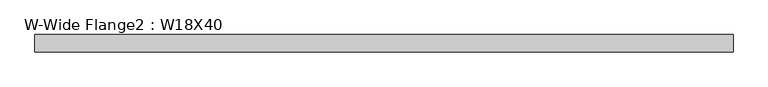
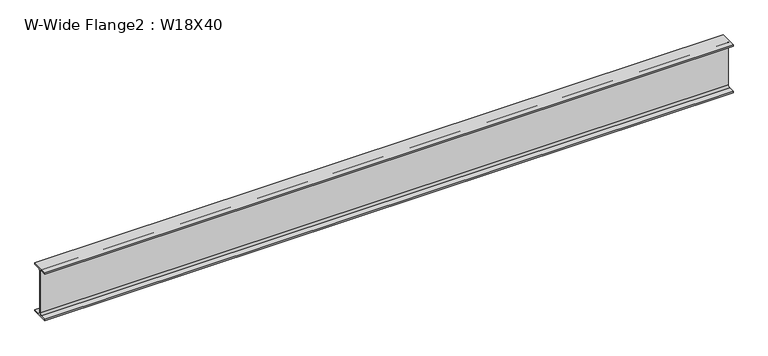
"""IFC4 building model written with IfcOpenShell, lengths in millimetres: beam geometry, W-Wide Flange2 : W18X40."""

import ifcopenshell
import ifcopenshell.guid

model = None  # the IFC model being written
_history = None  # IfcOwnerHistory: only IFC2X3 demands one
_inside = {}  # id of a spatial element -> (the spatial element, [elements in it])
_under = {}  # id of a project, library or spatial element -> (it, [spatial elements below it])
_declared = {}  # id of a project -> (the project, [libraries it declares])
_typed = {}  # id of a type object -> (the type object, [elements of that type])
_made_of = {}  # id of a material, layer set ... -> (it, [elements and type objects made of it])


def new_model(schema):
    """Start an empty IFC model of exactly this schema.

    Asked for "IFC4X3", IfcOpenShell would pick the latest addendum, in which some entities
    have other attributes; the version numbers below select the first issue.
    IFC2X3 requires an IfcOwnerHistory on every rooted entity: one is made here for all.
    """
    global model, _history
    if schema == "IFC4X3":
        model = ifcopenshell.file(schema_version=(4, 3, 0, 0))
    else:
        model = ifcopenshell.file(schema=schema)
    _inside.clear()
    _under.clear()
    _declared.clear()
    _typed.clear()
    _made_of.clear()
    _history = None
    if model.schema == "IFC2X3":
        org = make("IfcOrganization", Name="unknown")
        user = make(
            "IfcPersonAndOrganization",
            ThePerson=make("IfcPerson", FamilyName="unknown"),
            TheOrganization=org,
        )
        app = make(
            "IfcApplication",
            ApplicationDeveloper=org,
            Version="unknown",
            ApplicationFullName="unknown",
            ApplicationIdentifier="unknown",
        )
        _history = make(
            "IfcOwnerHistory",
            OwningUser=user,
            OwningApplication=app,
            ChangeAction="ADDED",
            CreationDate=0,
        )
    return model


def make(cls, **values):
    """One entity of the class cls with the attributes given. An attribute that is None is left unset."""
    return model.create_entity(
        cls, **{name: value for name, value in values.items() if value is not None}
    )


def rooted(cls, **values):
    """An entity with a GlobalId (a new one), such as an element, a storey or a relation."""
    return make(cls, GlobalId=ifcopenshell.guid.new(), OwnerHistory=_history, **values)


def si_unit(unit_type, name, prefix=None):
    """IfcSIUnit, for example si_unit("LENGTHUNIT", "METRE", prefix="MILLI")."""
    return make("IfcSIUnit", UnitType=unit_type, Prefix=prefix, Name=name)


def assignment(units):
    """IfcUnitAssignment: the units of a project."""
    return None if units is None else make("IfcUnitAssignment", Units=units)


def point(xyz):
    """IfcCartesianPoint."""
    return None if xyz is None else make("IfcCartesianPoint", Coordinates=xyz)


def direction(xyz):
    """IfcDirection."""
    return None if xyz is None else make("IfcDirection", DirectionRatios=xyz)


def frame(location, z_axis=None, x_axis=None):
    """IfcAxis2Placement3D, a coordinate frame: its origin and axes. An axis left out is left unset."""
    return make(
        "IfcAxis2Placement3D",
        Location=point(location),
        Axis=direction(z_axis),
        RefDirection=direction(x_axis),
    )


def frame_2d(location, x_axis=None):
    """IfcAxis2Placement2D, a coordinate frame in the plane: its origin and x axis."""
    return make(
        "IfcAxis2Placement2D", Location=point(location), RefDirection=direction(x_axis)
    )


def origin():
    """The frame at (0, 0, 0) with its axes left unset."""
    return frame((0.0, 0.0, 0.0))


def place(relative_to, where):
    """IfcLocalPlacement: puts the frame where relative to a parent placement (None: the world)."""
    return make(
        "IfcLocalPlacement", PlacementRelTo=relative_to, RelativePlacement=where
    )


def context(
    kind, dimensions, precision=None, world=None, true_north=None, identifier=None
):
    """IfcGeometricRepresentationContext, for example the 3D "Model" context."""
    return make(
        "IfcGeometricRepresentationContext",
        ContextIdentifier=identifier,
        ContextType=kind,
        CoordinateSpaceDimension=dimensions,
        Precision=precision,
        WorldCoordinateSystem=world,
        TrueNorth=true_north,
    )


def project(units=None, contexts=None):
    """IfcProject with its units and contexts."""
    return rooted(
        "IfcProject",
        Name="project",
        RepresentationContexts=contexts,
        UnitsInContext=assignment(units),
    )


def spatial(cls, under=None, at=None, **own):
    """A site, building, storey or space (cls), placed at a placement, below another one or the project."""
    s = rooted(cls, ObjectPlacement=at, **own)
    if under is not None:
        _under.setdefault(under.id(), (under, []))[1].append(s)
    return s


def polyline(points):
    """IfcPolyline through the points."""
    return make("IfcPolyline", Points=[point(p) for p in points])


def circle_curve(where, radius):
    """IfcCircle in the frame where."""
    return make("IfcCircle", Position=where, Radius=radius)


def trimmed(basis, trim1, trim2, sense, master):
    """IfcTrimmedCurve: the piece of a basis curve between two trims."""
    return make(
        "IfcTrimmedCurve",
        BasisCurve=basis,
        Trim1=trim1,
        Trim2=trim2,
        SenseAgreement=sense,
        MasterRepresentation=master,
    )


def segment(curve, same_sense, transition):
    """IfcCompositeCurveSegment."""
    return make(
        "IfcCompositeCurveSegment",
        Transition=transition,
        SameSense=same_sense,
        ParentCurve=curve,
    )


def composite_curve(segments, self_intersect=None):
    """IfcCompositeCurve: segments joined end to end."""
    return make("IfcCompositeCurve", Segments=segments, SelfIntersect=self_intersect)


def outline(outer, holes=None, kind="AREA"):
    """IfcArbitraryClosedProfileDef: a profile drawn as a closed curve; with holes, ...WithVoids."""
    if holes is None:
        return make("IfcArbitraryClosedProfileDef", ProfileType=kind, OuterCurve=outer)
    return make(
        "IfcArbitraryProfileDefWithVoids",
        ProfileType=kind,
        OuterCurve=outer,
        InnerCurves=holes,
    )


def extrude(swept, where, along, depth):
    """IfcExtrudedAreaSolid: the profile swept, set in the frame where, extruded along a direction by depth."""
    return make(
        "IfcExtrudedAreaSolid",
        SweptArea=swept,
        Position=where,
        ExtrudedDirection=direction(along),
        Depth=depth,
    )


def shape(context_of_items, identifier, shape_type, items):
    """IfcShapeRepresentation: the items that make up one representation, for example the "Body"."""
    return make(
        "IfcShapeRepresentation",
        ContextOfItems=context_of_items,
        RepresentationIdentifier=identifier,
        RepresentationType=shape_type,
        Items=items,
    )


def source(mapping_origin, context_of_items, identifier, shape_type, items):
    """IfcRepresentationMap: a shape defined once, which mapped items show again and again."""
    return make(
        "IfcRepresentationMap",
        MappingOrigin=mapping_origin,
        MappedRepresentation=shape(context_of_items, identifier, shape_type, items),
    )


def transform(
    local_origin,
    x_axis=None,
    y_axis=None,
    z_axis=None,
    scale=None,
    scale2=None,
    scale3=None,
    uniform=True,
):
    """IfcCartesianTransformationOperator3D, or its non-uniform kind. x_axis, y_axis, z_axis: its Axis1, 2, 3."""
    if uniform:
        return make(
            "IfcCartesianTransformationOperator3D",
            Axis1=direction(x_axis),
            Axis2=direction(y_axis),
            LocalOrigin=point(local_origin),
            Scale=scale,
            Axis3=direction(z_axis),
        )
    return make(
        "IfcCartesianTransformationOperator3DnonUniform",
        Axis1=direction(x_axis),
        Axis2=direction(y_axis),
        LocalOrigin=point(local_origin),
        Scale=scale,
        Axis3=direction(z_axis),
        Scale2=scale2,
        Scale3=scale3,
    )


def mapped(mapping_source, mapping_target):
    """IfcMappedItem: shows the shape of a source again, moved by a transform."""
    return make(
        "IfcMappedItem", MappingSource=mapping_source, MappingTarget=mapping_target
    )


def made_of(thing, what):
    """Note that an element or type object is made of a material, layer set ...; save() writes the relation."""
    if what is not None:
        _made_of.setdefault(what.id(), (what, []))[1].append(thing)
    return thing


def element(
    cls,
    number,
    at=None,
    inside=None,
    cuts=None,
    type_object=None,
    material=None,
    context=None,
    identifier="Body",
    shape_type=None,
    held_by="IfcProductDefinitionShape",
    body=None,
    shapes=None,
    **own,
):
    """One element of the class cls, such as IfcWall. Its Tag is "e" and its number.

    at: its placement. inside: the storey or other place that contains it. cuts: it is an
    opening in that element (IfcRelVoidsElement). A single representation is given by context,
    identifier, shape_type and body (its items); several are given by shapes. held_by: the class
    of the entity that holds the representations. save() writes the other relations.
    """
    e = rooted(cls, Tag="e%d" % number, ObjectPlacement=at, **own)
    if body is not None:
        shapes = [shape(context, identifier, shape_type, body)]
    if shapes is not None:
        e.Representation = make(held_by, Representations=shapes)
    if inside is not None:
        _inside.setdefault(inside.id(), (inside, []))[1].append(e)
    if cuts is not None:
        rooted(
            "IfcRelVoidsElement", RelatingBuildingElement=cuts, RelatedOpeningElement=e
        )
    if type_object is not None:
        _typed.setdefault(type_object.id(), (type_object, []))[1].append(e)
    return made_of(e, material)


def aggregate(whole, parts):
    """IfcRelAggregates: a whole, such as a stair, and the parts it consists of."""
    return rooted("IfcRelAggregates", RelatingObject=whole, RelatedObjects=parts)


def save(model, path):
    """Write the relations noted so far, then the file.

    IfcRelAggregates (storeys below a building ...), IfcRelContainedInSpatialStructure (elements
    in a storey), IfcRelDefinesByType, IfcRelAssociatesMaterial and IfcRelDeclares: one each for
    every whole, place, type object, material and project.
    """
    for whole, parts in _under.values():
        aggregate(whole, parts)
    for where, things in _inside.values():
        rooted(
            "IfcRelContainedInSpatialStructure",
            RelatedElements=things,
            RelatingStructure=where,
        )
    for kind, things in _typed.values():
        rooted("IfcRelDefinesByType", RelatedObjects=things, RelatingType=kind)
    for what, things in _made_of.values():
        rooted("IfcRelAssociatesMaterial", RelatedObjects=things, RelatingMaterial=what)
    for by, libraries in _declared.values():
        rooted("IfcRelDeclares", RelatingContext=by, RelatedDefinitions=libraries)
    model.write(path)


def w_wide_flange2_w18x40_30b59f7b(model_context):
    return source(origin(), model_context, "Body", "SweptSolid", [
        extrude(outline(composite_curve([segment(polyline([(76.454, -213.995), (76.454, -227.33), (-76.454, -227.33), (-76.454, -213.995), (-20.828, -213.995)]), True, "CONTINUOUS"), segment(trimmed(circle_curve(frame_2d((-20.828, -197.1675)), 16.8275), [point((-20.828, -213.995))], [point((-4.0005, -197.1675))], True, "CARTESIAN"), True, "CONTINUOUS"), segment(polyline([(-4.0005, -197.1675), (-4.0005, 197.1675)]), True, "CONTINUOUS"), segment(trimmed(circle_curve(frame_2d((-20.828, 197.1675)), 16.8275), [point((-4.0005, 197.1675))], [point((-20.828, 213.995))], True, "CARTESIAN"), True, "CONTINUOUS"), segment(polyline([(-20.828, 213.995), (-76.454, 213.995), (-76.454, 227.33), (76.454, 227.33), (76.454, 213.995), (20.828, 213.995)]), True, "CONTINUOUS"), segment(trimmed(circle_curve(frame_2d((20.828, 197.1675)), 16.8275), [point((20.828, 213.995))], [point((4.0005, 197.1675))], True, "CARTESIAN"), True, "CONTINUOUS"), segment(polyline([(4.0005, 197.1675), (4.0005, -197.1675)]), True, "CONTINUOUS"), segment(trimmed(circle_curve(frame_2d((20.828, -197.1675)), 16.8275), [point((4.0005, -197.1675))], [point((20.828, -213.995))], True, "CARTESIAN"), True, "CONTINUOUS"), segment(polyline([(20.828, -213.995), (76.454, -213.995)]), True, "CONTINUOUS")], self_intersect=False)), frame((-3079.353125, 0.0, 0.0), z_axis=(1.0, 0.0, 0.0), x_axis=(0.0, 1.0, 0.0)), (0.0, 0.0, 1.0), 6158.70625),
    ])


if __name__ == "__main__":
    model = new_model("IFC4")
    model_context = context("Model", 3, world=origin())
    ifc_project = project(units=[si_unit("LENGTHUNIT", "METRE", prefix="MILLI")], contexts=[model_context])
    site = spatial("IfcSite", under=ifc_project)
    building = spatial("IfcBuilding", under=site)
    placement = place(None, origin())
    w_wide_flange2_w18x40_shape = w_wide_flange2_w18x40_30b59f7b(model_context)
    element("IfcBeam", 1, ObjectType="W-Wide Flange2 : W18X40", at=placement, inside=building, context=model_context, shape_type="MappedRepresentation", body=[
        mapped(w_wide_flange2_w18x40_shape, transform((0.0, 0.0, 0.0), x_axis=(1.0, 0.0, 0.0), y_axis=(0.0, 1.0, 0.0), z_axis=(0.0, 0.0, 1.0))),
    ])
    save(model, "model.ifc")

# Revit data of these elements
# Type "W-Wide Flange2 : W18X40"
#   Assembly Code = "B10"
#   W = 40
#   Length [instance default] = 5' - 0"
#   bf = 0' - 6.02"
#   d = 1' - 5.9"
#   k = 0' - 1 3/16"
#   k2 = 0' - 0.6625"
#   tf = 0' - 0.525"
#   tw = 0' - 0.315"
#   A = 0.0819444 SF
#   Structural Material [instance default] = Steel ASTM A992
# Element 1 (IfcBeam, "W-Wide Flange2 : W18X40")
#   Materials on its faces: "Steel ASTM A992"
# Materials
#   "Steel ASTM A992": class "Metal", colour RGB 199 199 199, transparency 0, Description = "Structural steel 50ksi", Cost = 0
